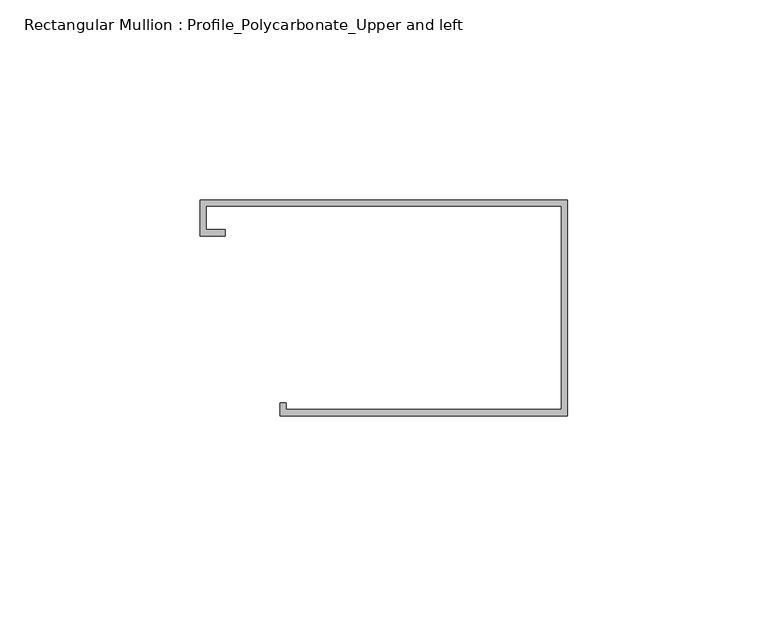
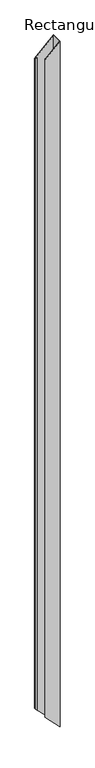
"""IFC4 building model written with IfcOpenShell, lengths in millimetres: member geometry, Rectangular Mullion : Profile_Polycarbonate_Upper and left."""

import ifcopenshell
import ifcopenshell.guid

model = None  # the IFC model being written
_history = None  # IfcOwnerHistory: only IFC2X3 demands one
_inside = {}  # id of a spatial element -> (the spatial element, [elements in it])
_under = {}  # id of a project, library or spatial element -> (it, [spatial elements below it])
_declared = {}  # id of a project -> (the project, [libraries it declares])
_typed = {}  # id of a type object -> (the type object, [elements of that type])
_made_of = {}  # id of a material, layer set ... -> (it, [elements and type objects made of it])


def new_model(schema):
    """Start an empty IFC model of exactly this schema.

    Asked for "IFC4X3", IfcOpenShell would pick the latest addendum, in which some entities
    have other attributes; the version numbers below select the first issue.
    IFC2X3 requires an IfcOwnerHistory on every rooted entity: one is made here for all.
    """
    global model, _history
    if schema == "IFC4X3":
        model = ifcopenshell.file(schema_version=(4, 3, 0, 0))
    else:
        model = ifcopenshell.file(schema=schema)
    _inside.clear()
    _under.clear()
    _declared.clear()
    _typed.clear()
    _made_of.clear()
    _history = None
    if model.schema == "IFC2X3":
        org = make("IfcOrganization", Name="unknown")
        user = make(
            "IfcPersonAndOrganization",
            ThePerson=make("IfcPerson", FamilyName="unknown"),
            TheOrganization=org,
        )
        app = make(
            "IfcApplication",
            ApplicationDeveloper=org,
            Version="unknown",
            ApplicationFullName="unknown",
            ApplicationIdentifier="unknown",
        )
        _history = make(
            "IfcOwnerHistory",
            OwningUser=user,
            OwningApplication=app,
            ChangeAction="ADDED",
            CreationDate=0,
        )
    return model


def make(cls, **values):
    """One entity of the class cls with the attributes given. An attribute that is None is left unset."""
    return model.create_entity(
        cls, **{name: value for name, value in values.items() if value is not None}
    )


def rooted(cls, **values):
    """An entity with a GlobalId (a new one), such as an element, a storey or a relation."""
    return make(cls, GlobalId=ifcopenshell.guid.new(), OwnerHistory=_history, **values)


def si_unit(unit_type, name, prefix=None):
    """IfcSIUnit, for example si_unit("LENGTHUNIT", "METRE", prefix="MILLI")."""
    return make("IfcSIUnit", UnitType=unit_type, Prefix=prefix, Name=name)


def assignment(units):
    """IfcUnitAssignment: the units of a project."""
    return None if units is None else make("IfcUnitAssignment", Units=units)


def point(xyz):
    """IfcCartesianPoint."""
    return None if xyz is None else make("IfcCartesianPoint", Coordinates=xyz)


def direction(xyz):
    """IfcDirection."""
    return None if xyz is None else make("IfcDirection", DirectionRatios=xyz)


def frame(location, z_axis=None, x_axis=None):
    """IfcAxis2Placement3D, a coordinate frame: its origin and axes. An axis left out is left unset."""
    return make(
        "IfcAxis2Placement3D",
        Location=point(location),
        Axis=direction(z_axis),
        RefDirection=direction(x_axis),
    )


def origin():
    """The frame at (0, 0, 0) with its axes left unset."""
    return frame((0.0, 0.0, 0.0))


def place(relative_to, where):
    """IfcLocalPlacement: puts the frame where relative to a parent placement (None: the world)."""
    return make(
        "IfcLocalPlacement", PlacementRelTo=relative_to, RelativePlacement=where
    )


def context(
    kind, dimensions, precision=None, world=None, true_north=None, identifier=None
):
    """IfcGeometricRepresentationContext, for example the 3D "Model" context."""
    return make(
        "IfcGeometricRepresentationContext",
        ContextIdentifier=identifier,
        ContextType=kind,
        CoordinateSpaceDimension=dimensions,
        Precision=precision,
        WorldCoordinateSystem=world,
        TrueNorth=true_north,
    )


def project(units=None, contexts=None):
    """IfcProject with its units and contexts."""
    return rooted(
        "IfcProject",
        Name="project",
        RepresentationContexts=contexts,
        UnitsInContext=assignment(units),
    )


def spatial(cls, under=None, at=None, **own):
    """A site, building, storey or space (cls), placed at a placement, below another one or the project."""
    s = rooted(cls, ObjectPlacement=at, **own)
    if under is not None:
        _under.setdefault(under.id(), (under, []))[1].append(s)
    return s


def faces_of(points, faces, orient=None, outer=None):
    """IfcFace entities. A face is a list of loops; a loop is a list of indices into points, from 0.

    orient and outer hold one flag for each loop. By default every Orientation is true, the
    first loop of a face is its IfcFaceOuterBound and the others are IfcFaceBound.
    """
    made = []
    for i, loops in enumerate(faces):
        bounds = []
        for j, loop in enumerate(loops):
            is_outer = j == 0 if outer is None else outer[i][j]
            bounds.append(
                make(
                    "IfcFaceOuterBound" if is_outer else "IfcFaceBound",
                    Bound=make("IfcPolyLoop", Polygon=[points[k] for k in loop]),
                    Orientation=True if orient is None else orient[i][j],
                )
            )
        made.append(make("IfcFace", Bounds=bounds))
    return made


def faceted_brep(points, faces, orient=None, outer=None, voids=None):
    """IfcFacetedBrep: a solid bounded by flat faces; with voids (closed shells), ...WithVoids."""
    shared = [point(p) for p in points]
    hull = make("IfcClosedShell", CfsFaces=faces_of(shared, faces, orient, outer))
    if voids is None:
        return make("IfcFacetedBrep", Outer=hull)
    return make(
        "IfcFacetedBrepWithVoids",
        Outer=hull,
        Voids=[
            make(cls, CfsFaces=faces_of(shared, fs, o, b)) for cls, fs, o, b in voids
        ],
    )


def shape(context_of_items, identifier, shape_type, items):
    """IfcShapeRepresentation: the items that make up one representation, for example the "Body"."""
    return make(
        "IfcShapeRepresentation",
        ContextOfItems=context_of_items,
        RepresentationIdentifier=identifier,
        RepresentationType=shape_type,
        Items=items,
    )


def source(mapping_origin, context_of_items, identifier, shape_type, items):
    """IfcRepresentationMap: a shape defined once, which mapped items show again and again."""
    return make(
        "IfcRepresentationMap",
        MappingOrigin=mapping_origin,
        MappedRepresentation=shape(context_of_items, identifier, shape_type, items),
    )


def transform(
    local_origin,
    x_axis=None,
    y_axis=None,
    z_axis=None,
    scale=None,
    scale2=None,
    scale3=None,
    uniform=True,
):
    """IfcCartesianTransformationOperator3D, or its non-uniform kind. x_axis, y_axis, z_axis: its Axis1, 2, 3."""
    if uniform:
        return make(
            "IfcCartesianTransformationOperator3D",
            Axis1=direction(x_axis),
            Axis2=direction(y_axis),
            LocalOrigin=point(local_origin),
            Scale=scale,
            Axis3=direction(z_axis),
        )
    return make(
        "IfcCartesianTransformationOperator3DnonUniform",
        Axis1=direction(x_axis),
        Axis2=direction(y_axis),
        LocalOrigin=point(local_origin),
        Scale=scale,
        Axis3=direction(z_axis),
        Scale2=scale2,
        Scale3=scale3,
    )


def mapped(mapping_source, mapping_target):
    """IfcMappedItem: shows the shape of a source again, moved by a transform."""
    return make(
        "IfcMappedItem", MappingSource=mapping_source, MappingTarget=mapping_target
    )


def made_of(thing, what):
    """Note that an element or type object is made of a material, layer set ...; save() writes the relation."""
    if what is not None:
        _made_of.setdefault(what.id(), (what, []))[1].append(thing)
    return thing


def element(
    cls,
    number,
    at=None,
    inside=None,
    cuts=None,
    type_object=None,
    material=None,
    context=None,
    identifier="Body",
    shape_type=None,
    held_by="IfcProductDefinitionShape",
    body=None,
    shapes=None,
    **own,
):
    """One element of the class cls, such as IfcWall. Its Tag is "e" and its number.

    at: its placement. inside: the storey or other place that contains it. cuts: it is an
    opening in that element (IfcRelVoidsElement). A single representation is given by context,
    identifier, shape_type and body (its items); several are given by shapes. held_by: the class
    of the entity that holds the representations. save() writes the other relations.
    """
    e = rooted(cls, Tag="e%d" % number, ObjectPlacement=at, **own)
    if body is not None:
        shapes = [shape(context, identifier, shape_type, body)]
    if shapes is not None:
        e.Representation = make(held_by, Representations=shapes)
    if inside is not None:
        _inside.setdefault(inside.id(), (inside, []))[1].append(e)
    if cuts is not None:
        rooted(
            "IfcRelVoidsElement", RelatingBuildingElement=cuts, RelatedOpeningElement=e
        )
    if type_object is not None:
        _typed.setdefault(type_object.id(), (type_object, []))[1].append(e)
    return made_of(e, material)


def aggregate(whole, parts):
    """IfcRelAggregates: a whole, such as a stair, and the parts it consists of."""
    return rooted("IfcRelAggregates", RelatingObject=whole, RelatedObjects=parts)


def save(model, path):
    """Write the relations noted so far, then the file.

    IfcRelAggregates (storeys below a building ...), IfcRelContainedInSpatialStructure (elements
    in a storey), IfcRelDefinesByType, IfcRelAssociatesMaterial and IfcRelDeclares: one each for
    every whole, place, type object, material and project.
    """
    for whole, parts in _under.values():
        aggregate(whole, parts)
    for where, things in _inside.values():
        rooted(
            "IfcRelContainedInSpatialStructure",
            RelatedElements=things,
            RelatingStructure=where,
        )
    for kind, things in _typed.values():
        rooted("IfcRelDefinesByType", RelatedObjects=things, RelatingType=kind)
    for what, things in _made_of.values():
        rooted("IfcRelAssociatesMaterial", RelatedObjects=things, RelatingMaterial=what)
    for by, libraries in _declared.values():
        rooted("IfcRelDeclares", RelatingContext=by, RelatedDefinitions=libraries)
    model.write(path)


def rectangular_mullion_profile_polycarbonate_upper_and_left_59b87f0f(model_context):
    return source(origin(), model_context, "Body", "Brep", [
        faceted_brep([(-91.9988, 28.984575, -88.2453421), (0.0, 28.984575, 0.0), (0.0, 28.984575, -3533.6634279), (-91.9988, 28.984575, -3437.7515191), (-91.9988, 19.992975, -88.2453421), (-91.9988, 19.992975, -3437.7515191), (-85.6488, 19.992975, -82.1544157), (-85.6488, 19.992975, -3444.3716122), (-85.6488, 21.580475, -82.1544157), (-85.6488, 21.580475, -3444.3716122), (-90.4113, 21.580475, -86.7226105), (-90.4113, 21.580475, -3439.4065424), (-90.4113, 27.397075, -86.7226105), (-90.4113, 27.397075, -3439.4065424), (-1.5875, 27.397075, -1.5227316), (-1.5875, 27.397075, -3532.0084046), (-1.5875, -23.428325, -1.5227316), (-1.5875, -23.428325, -3532.0084046), (-70.3961, -23.428325, -67.5240104), (-70.3961, -23.428325, -3460.2730758), (-70.3961, -21.840825, -67.5240104), (-70.3961, -21.840825, -3460.2730758), (-71.9836, -21.840825, -69.046742), (-71.9836, -21.840825, -3458.6180526), (-71.9836, -25.015825, -69.046742), (-71.9836, -25.015825, -3458.6180526), (0.0, -25.015825, 0.0), (0.0, -25.015825, -3533.6634279)], [[[0, 1, 2, 3]], [[4, 0, 3, 5]], [[6, 4, 5, 7]], [[8, 6, 7, 9]], [[10, 8, 9, 11]], [[12, 10, 11, 13]], [[14, 12, 13, 15]], [[16, 14, 15, 17]], [[18, 16, 17, 19]], [[20, 18, 19, 21]], [[22, 20, 21, 23]], [[24, 22, 23, 25]], [[26, 24, 25, 27]], [[1, 26, 27, 2]], [[1, 0, 4, 6, 8, 10, 12, 14, 16, 18, 20, 22, 24, 26]], [[2, 27, 25, 23, 21, 19, 17, 15, 13, 11, 9, 7, 5, 3]]]),
    ])


if __name__ == "__main__":
    model = new_model("IFC4")
    model_context = context("Model", 3, world=origin())
    ifc_project = project(units=[si_unit("LENGTHUNIT", "METRE", prefix="MILLI")], contexts=[model_context])
    site = spatial("IfcSite", under=ifc_project)
    building = spatial("IfcBuilding", under=site)
    placement = place(None, origin())
    rectangular_mullion_profile_polycarbonate_upper_and_left_shape = rectangular_mullion_profile_polycarbonate_upper_and_left_59b87f0f(model_context)
    element("IfcMember", 1, ObjectType="Rectangular Mullion : Profile_Polycarbonate_Upper and left", at=placement, inside=building, context=model_context, shape_type="MappedRepresentation", body=[
        mapped(rectangular_mullion_profile_polycarbonate_upper_and_left_shape, transform((0.0, 0.0, 0.0), x_axis=(1.0, 0.0, 0.0), y_axis=(0.0, 1.0, 0.0), z_axis=(0.0, 0.0, 1.0))),
    ])
    save(model, "model.ifc")

# Revit data of these elements
# Type "Rectangular Mullion : Profile_Polycarbonate_Upper and left"
#   built-in parameter 1007322 = 0.177167 (stored number, unit not read)
#   built-in parameter 1007321 = 0.00520833 (stored number, unit not read)
#   built-in parameter 1007320 = 0 (stored number, unit not read)
